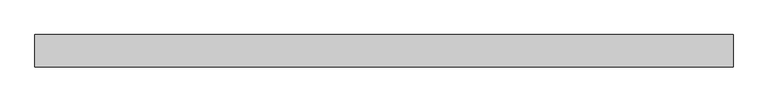
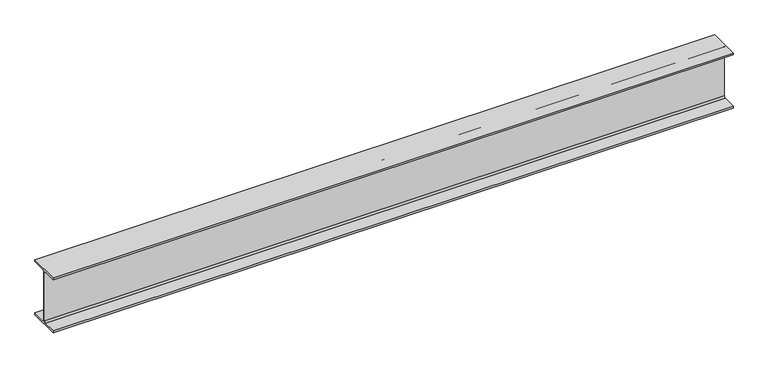
"""IFC4 building model written with IfcOpenShell, lengths in millimetres: beam geometry, Old_Steel Beam_H-KSD3502 : H_SB_ASB_H-200×200x8x12."""

from ifc_helpers import new_model, si_unit, point, frame, frame_2d, origin, place, context, project, spatial, polyline, circle_curve, trimmed, segment, composite_curve, outline, extrude, source, transform, mapped, element, save


def beam_588beb59(model_context):
    return source(origin(), model_context, "Body", "SweptSolid", [
        extrude(outline(composite_curve([segment(polyline([(82.5, -141.5), (82.5, -151.7), (-82.5, -151.7), (-82.5, -141.5), (-11.9, -141.5)]), True, "CONTINUOUS"), segment(trimmed(circle_curve(frame_2d((-11.9, -132.6)), 8.9), [point((-11.9, -141.5))], [point((-3.0, -132.6))], True, "CARTESIAN"), True, "CONTINUOUS"), segment(polyline([(-3.0, -132.6), (-3.0, 132.6)]), True, "CONTINUOUS"), segment(trimmed(circle_curve(frame_2d((-11.9, 132.6)), 8.9), [point((-3.0, 132.6))], [point((-11.9, 141.5))], True, "CARTESIAN"), True, "CONTINUOUS"), segment(polyline([(-11.9, 141.5), (-82.5, 141.5), (-82.5, 151.7), (82.5, 151.7), (82.5, 141.5), (11.9, 141.5)]), True, "CONTINUOUS"), segment(trimmed(circle_curve(frame_2d((11.9, 132.6)), 8.9), [point((11.9, 141.5))], [point((3.0, 132.6))], True, "CARTESIAN"), True, "CONTINUOUS"), segment(polyline([(3.0, 132.6), (3.0, -132.6)]), True, "CONTINUOUS"), segment(trimmed(circle_curve(frame_2d((11.9, -132.6)), 8.9), [point((3.0, -132.6))], [point((11.9, -141.5))], True, "CARTESIAN"), True, "CONTINUOUS"), segment(polyline([(11.9, -141.5), (82.5, -141.5)]), True, "CONTINUOUS")], self_intersect=False)), frame((-1835.8461272, 0.0, 0.0), z_axis=(1.0, 0.0, 0.0), x_axis=(0.0, 1.0, 0.0)), (0.0, 0.0, 1.0), 3545.7762812),
    ])


if __name__ == "__main__":
    model = new_model("IFC4")
    model_context = context("Model", 3, world=origin())
    ifc_project = project(units=[si_unit("LENGTHUNIT", "METRE", prefix="MILLI")], contexts=[model_context])
    site = spatial("IfcSite", under=ifc_project)
    building = spatial("IfcBuilding", under=site)
    placement = place(None, origin())
    beam_shape = beam_588beb59(model_context)
    element("IfcBeam", 1, ObjectType="Old_Steel Beam_H-KSD3502 : H_SB_ASB_H-200×200x8x12", at=placement, inside=building, context=model_context, shape_type="MappedRepresentation", body=[
        mapped(beam_shape, transform((0.0, 0.0, 0.0), x_axis=(1.0, 0.0, 0.0), y_axis=(0.0, 1.0, 0.0), z_axis=(0.0, 0.0, 1.0))),
    ])
    save(model, "model.ifc")

# Revit data of these elements
# Type "Old_Steel Beam_H-KSD3502 : H_SB_ASB_H-200×200x8x12"
#   Width = 20.0 cm
#   Web Thickness = 0.8 cm
#   Web Fillet = 1.3 cm
#   Warping Constant = 141376.0 cm⁶
#   Torsional Moment of Inertia = 26.2485 cm⁴
#   Torsional Modulus = 1.0 cm³
#   Section Area = 63.53 cm²
#   Plastic Modulus weak axis = 244.0 cm³
#   Plastic Modulus strong axis = 525.0 cm³
#   Perimeter = 1.16 m²/m
#   Nominal Weight = 49.90 kgf/m
#   Moment of Inertia weak axis = 1600.00 cm⁴
#   Moment of Inertia strong axis = 4720.00 cm⁴
#   Height = 20.0 cm
#   Flange Thickness = 1.2 cm
#   Elastic Modulus weak axis = 160.0 cm³
#   Elastic Modulus strong axis = 472.0 cm³
#   Centroid Vertical = 10.0 cm
#   Centroid Horizontal = 10.0 cm
#   Length [instance default] = 1.5240 m
#   Structural Material [instance default] = Steel, 45-345
#   Assembly Code = ""
# Element 1 (IfcBeam, "Old_Steel Beam_H-KSD3502 : H_SB_ASB_H-200×200x8x12")
#   Structural Material = none
# Materials
#   "Steel, 45-345": class "Metal", colour RGB 189 187 185, transparency 0, Description = "Steel 345 MPa", Cost = 0
